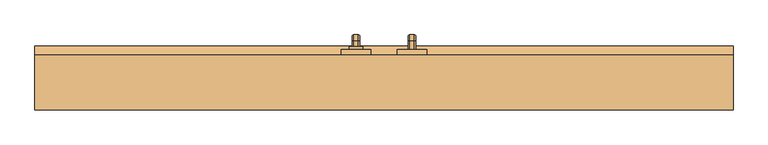
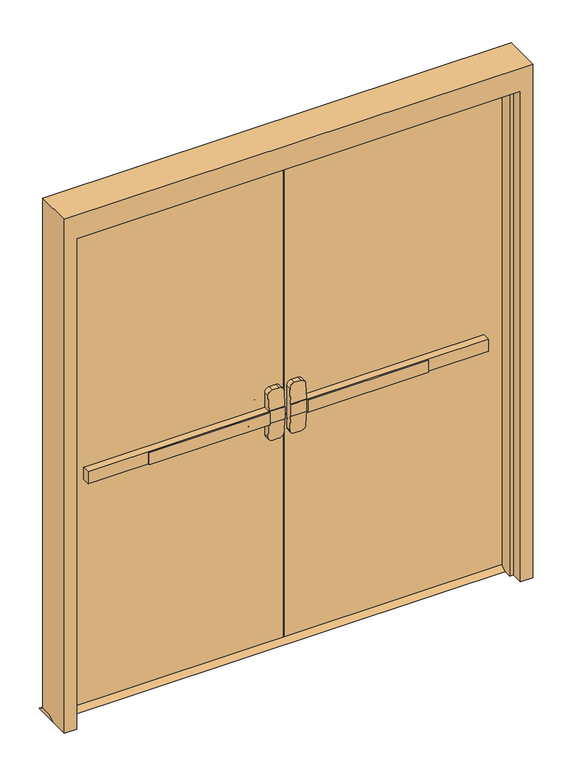
"""IFC4 building model written with IfcOpenShell, lengths in millimetres: door geometry, Дверь-Наружная-Двойная : Дверь-Наружная-Двойная."""

from ifc_helpers import new_model, si_unit, point, frame, frame_2d, origin, place, context, project, spatial, polyline, circle_curve, ellipse_curve, trimmed, segment, composite_curve, outline, extrude, faceted_brep, source, transform, mapped, element, save
from ifc_brep_helpers import plane_surface, cylinder_surface, revolved_surface, advanced_brep


def door_0e195155(model_context):
    return source(origin(), model_context, "Body", "SolidModel", [
        extrude(outline(polyline([(-566.1333333, -1.75), (-566.1333333, 4.6), (-76.2, 4.6), (-76.2, -1.75), (-566.1333333, -1.75)])), frame((0.0, 0.0, 974.6), z_axis=(0.0, 0.0, 1.0), x_axis=(1.0, 0.0, 0.0)), (0.0, 0.0, 1.0), 50.8),
        advanced_brep(
        [(-12.7, 4.6, 1025.4), (-76.2, 4.6, 1025.4), (-811.1, 4.6, 1025.4), (-811.1, 4.6, 974.6), (-76.2, 4.6, 974.6), (-12.7, 4.6, 974.6), (-811.1, 36.35, 1025.4), (-76.2, 36.35, 1025.4), (-76.2, 36.35, 1088.9), (-57.15, 36.35, 1107.95), (-31.75, 36.35, 1107.95), (-12.7, 36.35, 1088.9), (-12.7, 36.35, 911.1), (-31.75, 36.35, 892.05), (-57.15, 36.35, 892.05), (-76.2, 36.35, 911.1), (-76.2, 36.35, 974.6), (-811.1, 36.35, 974.6), (-12.7, 7.7752467, 1025.4), (-76.2, 7.7752467, 1025.4), (-12.7, 7.7752467, 974.6), (-12.7, 12.7854269, 911.1), (-12.7, 12.7854269, 1088.9), (-76.2, 7.7752467, 974.6), (-76.2, 12.7854269, 1088.9), (-76.2, 12.7854269, 911.1), (-57.15, 14.288481, 1107.95), (-31.75, 14.288481, 1107.95), (-31.75, 14.288481, 892.05), (-57.15, 14.288481, 892.05)],
        [
            (0, 1),
            (1, 2),
            (2, 3),
            (3, 4),
            (4, 5),
            (5, 0),
            (6, 7),
            (7, 8),
            (8, 9, circle_curve(frame((-57.15, 36.35, 1088.9), z_axis=(0.0, 1.0, 0.0), x_axis=(-1.0, 0.0, 0.0)), 19.05)),
            (9, 10),
            (10, 11, circle_curve(frame((-31.75, 36.35, 1088.9), z_axis=(0.0, 1.0, 0.0), x_axis=(-1.0, 0.0, 0.0)), 19.05)),
            (11, 12),
            (12, 13, circle_curve(frame((-31.75, 36.35, 911.1), z_axis=(0.0, 1.0, 0.0), x_axis=(-1.0, 0.0, 0.0)), 19.05)),
            (13, 14),
            (14, 15, circle_curve(frame((-57.15, 36.35, 911.1), z_axis=(0.0, 1.0, 0.0), x_axis=(-1.0, 0.0, 0.0)), 19.05)),
            (15, 16),
            (16, 17),
            (17, 6),
            (0, 18),
            (18, 19),
            (19, 7),
            (6, 2),
            (5, 20),
            (20, 21),
            (21, 12),
            (11, 22),
            (22, 18),
            (16, 23),
            (23, 20),
            (3, 17),
            (19, 24),
            (24, 8),
            (15, 25),
            (25, 23),
            (9, 26),
            (26, 27),
            (27, 10),
            (13, 28),
            (28, 29),
            (29, 14),
            (29, 25, ellipse_curve(frame((-57.15, 12.7854269, 911.1), z_axis=(0.0, 0.9969018152893365, 0.07865602756830282), x_axis=(0.0, -0.07865602756830208, 0.9969018152893365)), 19.1092038, 19.05)),
            (24, 26, ellipse_curve(frame((-57.15, 12.7854269, 1088.9), z_axis=(0.0, 0.9969018152893376, -0.07865602756828934), x_axis=(0.0, -0.078656027568288, -0.9969018152893377)), 19.1092038, 19.05)),
            (27, 22, ellipse_curve(frame((-31.75, 12.7854269, 1088.9), z_axis=(0.0, 0.9969018152893376, -0.07865602756828934), x_axis=(0.0, -0.078656027568288, -0.9969018152893377)), 19.1092038, 19.05)),
            (21, 28, ellipse_curve(frame((-31.75, 12.7854269, 911.1), z_axis=(0.0, 0.9969018152893365, 0.07865602756830282), x_axis=(0.0, -0.07865602756830208, 0.9969018152893365)), 19.1092038, 19.05)),
        ],
        [
            plane_surface(frame((-12.7, 4.6, 1025.4), z_axis=(0.0, -1.0, 0.0), x_axis=(1.0, 0.0, 0.0))),
            plane_surface(frame((-12.7, 36.35, 1025.4), z_axis=(0.0, 1.0, 0.0), x_axis=(-1.0, 0.0, 0.0))),
            plane_surface(frame((-811.1, 4.6, 1025.4), z_axis=(0.0, 0.0, 1.0), x_axis=(0.0, 1.0, 0.0))),
            plane_surface(frame((-12.7, 4.6, 1025.4), z_axis=(1.0, 0.0, 0.0), x_axis=(0.0, 1.0, 0.0))),
            plane_surface(frame((-12.7, 4.6, 974.6), z_axis=(0.0, 0.0, -1.0), x_axis=(0.0, 1.0, 0.0))),
            plane_surface(frame((-811.1, 4.6, 974.6), z_axis=(-1.0, 0.0, 0.0), x_axis=(0.0, 1.0, 0.0))),
            plane_surface(frame((-76.2, 7.7752467, 911.1), z_axis=(-1.0, 0.0, 0.0), x_axis=(0.0, 1.0, 0.0))),
            plane_surface(frame((-57.15, 7.7752467, 1107.95), z_axis=(0.0, 0.0, 1.0), x_axis=(0.0, 1.0, 0.0))),
            plane_surface(frame((-31.75, 7.7752467, 892.05), z_axis=(0.0, 0.0, -1.0), x_axis=(0.0, 1.0, 0.0))),
            cylinder_surface(frame((-57.15, 36.35, 911.1), z_axis=(0.0, -1.0, 0.0), x_axis=(-1.0, 0.0, 0.0)), 19.05),
            cylinder_surface(frame((-57.15, 36.35, 1088.9), z_axis=(0.0, -1.0, 0.0), x_axis=(-1.0, 0.0, 0.0)), 19.05),
            cylinder_surface(frame((-31.75, 36.35, 1088.9), z_axis=(0.0, -1.0, 0.0), x_axis=(-1.0, 0.0, 0.0)), 19.05),
            cylinder_surface(frame((-31.75, 36.35, 911.1), z_axis=(0.0, -1.0, 0.0), x_axis=(-1.0, 0.0, 0.0)), 19.05),
            plane_surface(frame((-76.2, 7.7752467, 1025.4), z_axis=(0.0, -0.9969018152893376, 0.07865602756828934), x_axis=(1.0, 0.0, 0.0))),
            plane_surface(frame((-76.2, 14.288481, 892.05), z_axis=(0.0, -0.9969018152893365, -0.07865602756830282), x_axis=(1.0, 0.0, 0.0))),
        ],
        [
            (0, [[1, 2, 3, 4, 5, 6]]),
            (1, [[7, 8, 9, 10, 11, 12, 13, 14, 15, 16, 17, 18]]),
            (2, [[-2, -1, 19, 20, 21, -7, 22]]),
            (3, [[23, 24, 25, -12, 26, 27, -19, -6]]),
            (4, [[-17, 28, 29, -23, -5, -4, 30]]),
            (5, [[-22, -18, -30, -3]]),
            (6, [[-21, 31, 32, -8]]),
            (6, [[33, 34, -28, -16]]),
            (7, [[35, 36, 37, -10]]),
            (8, [[38, 39, 40, -14]]),
            (9, [[-40, 41, -33, -15]]),
            (10, [[-32, 42, -35, -9]]),
            (11, [[-37, 43, -26, -11]]),
            (12, [[-25, 44, -38, -13]]),
            (13, [[-27, -43, -36, -42, -31, -20]]),
            (14, [[-29, -34, -41, -39, -44, -24]]),
        ],
    ),
        extrude(outline(polyline([(81.35, 15.0), (106.75, 0.0), (10.95, 0.0), (36.35, 15.0), (81.35, 15.0)])), frame((-950.0, 0.0, 0.0), z_axis=(1.0, 0.0, 0.0), x_axis=(0.0, 1.0, 0.0)), (0.0, 0.0, 1.0), 1900.0),
        extrude(outline(polyline([(566.1333333, -1.75), (76.2, -1.75), (76.2, 4.6), (566.1333333, 4.6), (566.1333333, -1.75)])), frame((0.0, 0.0, 974.6), z_axis=(0.0, 0.0, 1.0), x_axis=(1.0, 0.0, 0.0)), (0.0, 0.0, 1.0), 50.8),
        advanced_brep(
        [(12.7, 4.6, 1025.4), (12.7, 4.6, 974.6), (76.2, 4.6, 974.6), (811.1, 4.6, 974.6), (811.1, 4.6, 1025.4), (76.2, 4.6, 1025.4), (811.1, 36.35, 1025.4), (811.1, 36.35, 974.6), (76.2, 36.35, 974.6), (76.2, 36.35, 911.1), (57.15, 36.35, 892.05), (31.75, 36.35, 892.05), (12.7, 36.35, 911.1), (12.7, 36.35, 1088.9), (31.75, 36.35, 1107.95), (57.15, 36.35, 1107.95), (76.2, 36.35, 1088.9), (76.2, 36.35, 1025.4), (76.2, 7.7752467, 1025.4), (12.7, 7.7752467, 1025.4), (12.7, 12.7854269, 1088.9), (12.7, 12.7854269, 911.1), (12.7, 7.7752467, 974.6), (76.2, 7.7752467, 974.6), (76.2, 12.7854269, 911.1), (76.2, 12.7854269, 1088.9), (31.75, 14.288481, 1107.95), (57.15, 14.288481, 1107.95), (57.15, 14.288481, 892.05), (31.75, 14.288481, 892.05)],
        [
            (0, 1),
            (1, 2),
            (2, 3),
            (3, 4),
            (4, 5),
            (5, 0),
            (6, 7),
            (7, 8),
            (8, 9),
            (9, 10, circle_curve(frame((57.15, 36.35, 911.1), z_axis=(0.0, 1.0, 0.0), x_axis=(1.0, 0.0, 0.0)), 19.05)),
            (10, 11),
            (11, 12, circle_curve(frame((31.75, 36.35, 911.1), z_axis=(0.0, 1.0, 0.0), x_axis=(1.0, 0.0, 0.0)), 19.05)),
            (12, 13),
            (13, 14, circle_curve(frame((31.75, 36.35, 1088.9), z_axis=(0.0, 1.0, 0.0), x_axis=(1.0, 0.0, 0.0)), 19.05)),
            (14, 15),
            (15, 16, circle_curve(frame((57.15, 36.35, 1088.9), z_axis=(0.0, 1.0, 0.0), x_axis=(1.0, 0.0, 0.0)), 19.05)),
            (16, 17),
            (17, 6),
            (4, 6),
            (17, 18),
            (18, 19),
            (19, 0),
            (19, 20),
            (20, 13),
            (12, 21),
            (21, 22),
            (22, 1),
            (7, 3),
            (22, 23),
            (23, 8),
            (23, 24),
            (24, 9),
            (16, 25),
            (25, 18),
            (14, 26),
            (26, 27),
            (27, 15),
            (10, 28),
            (28, 29),
            (29, 11),
            (24, 28, ellipse_curve(frame((57.15, 12.7854269, 911.1), z_axis=(0.0, 0.9969018152893365, 0.07865602756830282), x_axis=(0.0, -0.07865602756830208, 0.9969018152893365)), 19.1092038, 19.05)),
            (27, 25, ellipse_curve(frame((57.15, 12.7854269, 1088.9), z_axis=(0.0, 0.9969018152893376, -0.07865602756828934), x_axis=(0.0, -0.078656027568288, -0.9969018152893377)), 19.1092038, 19.05)),
            (20, 26, ellipse_curve(frame((31.75, 12.7854269, 1088.9), z_axis=(0.0, 0.9969018152893376, -0.07865602756828934), x_axis=(0.0, -0.078656027568288, -0.9969018152893377)), 19.1092038, 19.05)),
            (29, 21, ellipse_curve(frame((31.75, 12.7854269, 911.1), z_axis=(0.0, 0.9969018152893365, 0.07865602756830282), x_axis=(0.0, -0.07865602756830208, 0.9969018152893365)), 19.1092038, 19.05)),
        ],
        [
            plane_surface(frame((12.7, 4.6, 1025.4), z_axis=(0.0, -1.0, 0.0), x_axis=(-1.0, 0.0, 0.0))),
            plane_surface(frame((12.7, 36.35, 1025.4), z_axis=(0.0, 1.0, 0.0), x_axis=(1.0, 0.0, 0.0))),
            plane_surface(frame((811.1, 4.6, 1025.4), z_axis=(0.0, 0.0, 1.0), x_axis=(0.0, 1.0, 0.0))),
            plane_surface(frame((12.7, 4.6, 1025.4), z_axis=(-1.0, 0.0, 0.0), x_axis=(0.0, 1.0, 0.0))),
            plane_surface(frame((12.7, 4.6, 974.6), z_axis=(0.0, 0.0, -1.0), x_axis=(0.0, 1.0, 0.0))),
            plane_surface(frame((811.1, 4.6, 974.6), z_axis=(1.0, 0.0, 0.0), x_axis=(0.0, 1.0, 0.0))),
            plane_surface(frame((76.2, 7.7752467, 911.1), z_axis=(1.0, 0.0, 0.0), x_axis=(0.0, 1.0, 0.0))),
            plane_surface(frame((57.15, 7.7752467, 1107.95), z_axis=(0.0, 0.0, 1.0), x_axis=(0.0, 1.0, 0.0))),
            plane_surface(frame((31.75, 7.7752467, 892.05), z_axis=(0.0, 0.0, -1.0), x_axis=(0.0, 1.0, 0.0))),
            cylinder_surface(frame((57.15, 36.35, 911.1), z_axis=(0.0, -1.0, 0.0), x_axis=(1.0, 0.0, 0.0)), 19.05),
            cylinder_surface(frame((57.15, 36.35, 1088.9), z_axis=(0.0, -1.0, 0.0), x_axis=(1.0, 0.0, 0.0)), 19.05),
            cylinder_surface(frame((31.75, 36.35, 1088.9), z_axis=(0.0, -1.0, 0.0), x_axis=(1.0, 0.0, 0.0)), 19.05),
            cylinder_surface(frame((31.75, 36.35, 911.1), z_axis=(0.0, -1.0, 0.0), x_axis=(1.0, 0.0, 0.0)), 19.05),
            plane_surface(frame((76.2, 7.7752467, 1025.4), z_axis=(0.0, -0.9969018152893376, 0.07865602756828934), x_axis=(-1.0, 0.0, 0.0))),
            plane_surface(frame((76.2, 14.288481, 892.05), z_axis=(0.0, -0.9969018152893365, -0.07865602756830282), x_axis=(-1.0, 0.0, 0.0))),
        ],
        [
            (0, [[1, 2, 3, 4, 5, 6]]),
            (1, [[7, 8, 9, 10, 11, 12, 13, 14, 15, 16, 17, 18]]),
            (2, [[19, -18, 20, 21, 22, -6, -5]]),
            (3, [[-1, -22, 23, 24, -13, 25, 26, 27]]),
            (4, [[28, -3, -2, -27, 29, 30, -8]]),
            (5, [[-4, -28, -7, -19]]),
            (6, [[-9, -30, 31, 32]]),
            (6, [[-17, 33, 34, -20]]),
            (7, [[-15, 35, 36, 37]]),
            (8, [[-11, 38, 39, 40]]),
            (9, [[-10, -32, 41, -38]]),
            (10, [[-16, -37, 42, -33]]),
            (11, [[-14, -24, 43, -35]]),
            (12, [[-12, -40, 44, -25]]),
            (13, [[-21, -34, -42, -36, -43, -23]]),
            (14, [[-26, -44, -39, -41, -31, -29]]),
        ],
    ),
        advanced_brep(
        [(66.2, 94.05, 1001.190625), (66.2, 94.05, 998.809375), (69.771875, 94.05, 995.2375), (82.6284594, 94.05, 995.2375), (86.2, 94.05, 998.8090406), (86.2, 94.05, 1001.190625), (82.628125, 94.05, 1004.7625), (69.771875, 94.05, 1004.7625), (66.2, 94.05, 874.609375), (69.771875, 94.05, 871.0375), (82.628125, 94.05, 871.0375), (86.2, 94.05, 874.609375), (86.2, 94.05, 876.9909594), (82.6284594, 94.05, 880.5625), (69.771875, 94.05, 880.5625), (66.2, 94.05, 876.990625), (66.2, 119.45, 1001.190625), (66.2, 133.340625, 987.3), (66.2, 133.340625, 888.5), (66.2, 119.45, 874.609375), (66.2, 119.45, 876.990625), (66.2, 130.959375, 888.5), (66.2, 130.959375, 987.3), (66.2, 119.45, 998.809375), (69.771875, 119.45, 995.2375), (82.6284594, 119.45, 995.2375), (86.2, 119.45, 998.8090406), (86.2, 130.9590406, 987.3), (86.2, 130.9590406, 888.5), (86.2, 119.45, 876.9909594), (86.2, 119.45, 874.609375), (86.2, 133.340625, 888.5), (86.2, 133.340625, 987.3), (86.2, 119.45, 1001.190625), (82.628125, 119.45, 1004.7625), (69.771875, 119.45, 1004.7625), (69.771875, 127.3875, 987.3), (82.6284594, 127.3875, 987.3), (82.628125, 136.9125, 987.3), (69.771875, 136.9125, 987.3), (69.771875, 127.3875, 888.5), (82.6284594, 127.3875, 888.5), (82.628125, 136.9125, 888.5), (69.771875, 136.9125, 888.5), (69.771875, 119.45, 880.5625), (82.6284594, 119.45, 880.5625), (82.628125, 119.45, 871.0375), (69.771875, 119.45, 871.0375)],
        [
            (0, 1),
            (1, 2, circle_curve(frame((69.771875, 94.05, 998.809375), z_axis=(0.0, -1.0, 0.0), x_axis=(0.0, 0.0, 1.0)), 3.571875)),
            (2, 3),
            (3, 4, circle_curve(frame((82.6284594, 94.05, 998.8090406), z_axis=(0.0, -1.0, 0.0), x_axis=(0.0, 0.0, 1.0)), 3.5715406)),
            (4, 5),
            (5, 6, circle_curve(frame((82.628125, 94.05, 1001.190625), z_axis=(0.0, -1.0, 0.0), x_axis=(0.0, 0.0, 1.0)), 3.571875)),
            (6, 7),
            (7, 0, circle_curve(frame((69.771875, 94.05, 1001.190625), z_axis=(0.0, -1.0, 0.0), x_axis=(0.0, 0.0, 1.0)), 3.571875)),
            (8, 9, circle_curve(frame((69.771875, 94.05, 874.609375), z_axis=(0.0, -1.0, 0.0), x_axis=(0.0, 0.0, -1.0)), 3.571875)),
            (9, 10),
            (10, 11, circle_curve(frame((82.628125, 94.05, 874.609375), z_axis=(0.0, -1.0, 0.0), x_axis=(0.0, 0.0, -1.0)), 3.571875)),
            (11, 12),
            (12, 13, circle_curve(frame((82.6284594, 94.05, 876.9909594), z_axis=(0.0, -1.0, 0.0), x_axis=(0.0, 0.0, -1.0)), 3.5715406)),
            (13, 14),
            (14, 15, circle_curve(frame((69.771875, 94.05, 876.990625), z_axis=(0.0, -1.0, 0.0), x_axis=(0.0, 0.0, -1.0)), 3.571875)),
            (15, 8),
            (0, 16),
            (16, 17, circle_curve(frame((66.2, 119.45, 987.3), z_axis=(-1.0, 0.0, 0.0), x_axis=(0.0, 0.0, 1.0)), 13.890625)),
            (17, 18),
            (18, 19, circle_curve(frame((66.2, 119.45, 888.5), z_axis=(-1.0, 0.0, 0.0), x_axis=(0.0, 1.0, 0.0)), 13.890625)),
            (19, 8),
            (15, 20),
            (20, 21, circle_curve(frame((66.2, 119.45, 888.5), z_axis=(1.0, 0.0, 0.0), x_axis=(0.0, 1.0, 0.0)), 11.509375)),
            (21, 22),
            (22, 23, circle_curve(frame((66.2, 119.45, 987.3), z_axis=(1.0, 0.0, 0.0), x_axis=(0.0, 0.0, 1.0)), 11.509375)),
            (23, 1),
            (23, 24, circle_curve(frame((69.771875, 119.45, 998.809375), z_axis=(0.0, -1.0, 0.0), x_axis=(0.0, 0.0, 1.0)), 3.571875)),
            (24, 2),
            (24, 25),
            (25, 3),
            (25, 26, circle_curve(frame((82.6284594, 119.45, 998.8090406), z_axis=(0.0, -1.0, 0.0), x_axis=(0.0, 0.0, 1.0)), 3.5715406)),
            (26, 4),
            (26, 27, circle_curve(frame((86.2, 119.45, 987.3), z_axis=(-1.0, 0.0, 0.0), x_axis=(0.0, 0.0, 1.0)), 11.5090406)),
            (27, 28),
            (28, 29, circle_curve(frame((86.2, 119.45, 888.5), z_axis=(-1.0, 0.0, 0.0), x_axis=(0.0, 1.0, 0.0)), 11.5090406)),
            (29, 12),
            (11, 30),
            (30, 31, circle_curve(frame((86.2, 119.45, 888.5), z_axis=(1.0, 0.0, 0.0), x_axis=(0.0, 1.0, 0.0)), 13.890625)),
            (31, 32),
            (32, 33, circle_curve(frame((86.2, 119.45, 987.3), z_axis=(1.0, 0.0, 0.0), x_axis=(0.0, 0.0, 1.0)), 13.890625)),
            (33, 5),
            (33, 34, circle_curve(frame((82.628125, 119.45, 1001.190625), z_axis=(0.0, -1.0, 0.0), x_axis=(0.0, 0.0, 1.0)), 3.571875)),
            (34, 6),
            (34, 35),
            (35, 7),
            (35, 16, circle_curve(frame((69.771875, 119.45, 1001.190625), z_axis=(0.0, -1.0, 0.0), x_axis=(0.0, 0.0, 1.0)), 3.571875)),
            (36, 24, circle_curve(frame((69.771875, 119.45, 987.3), z_axis=(1.0, 0.0, 0.0), x_axis=(0.0, 0.0, 1.0)), 7.9375)),
            (22, 36, circle_curve(frame((69.771875, 130.959375, 987.3), z_axis=(0.0, 0.0, 1.0), x_axis=(0.0, 1.0, 0.0)), 3.571875)),
            (37, 25, circle_curve(frame((82.6284594, 119.45, 987.3), z_axis=(1.0, 0.0, 0.0), x_axis=(0.0, 0.0, 1.0)), 7.9375)),
            (36, 37),
            (37, 27, circle_curve(frame((82.6284594, 130.9590406, 987.3), z_axis=(0.0, 0.0, 1.0), x_axis=(0.0, 1.0, 0.0)), 3.5715406)),
            (38, 34, circle_curve(frame((82.628125, 119.45, 987.3), z_axis=(1.0, 0.0, 0.0), x_axis=(0.0, 0.0, 1.0)), 17.4625)),
            (32, 38, circle_curve(frame((82.628125, 133.340625, 987.3), z_axis=(0.0, 0.0, 1.0), x_axis=(0.0, 1.0, 0.0)), 3.571875)),
            (39, 35, circle_curve(frame((69.771875, 119.45, 987.3), z_axis=(1.0, 0.0, 0.0), x_axis=(0.0, 0.0, 1.0)), 17.4625)),
            (38, 39),
            (39, 17, circle_curve(frame((69.771875, 133.340625, 987.3), z_axis=(0.0, 0.0, 1.0), x_axis=(0.0, 1.0, 0.0)), 3.571875)),
            (21, 40, circle_curve(frame((69.771875, 130.959375, 888.5), z_axis=(0.0, 0.0, 1.0), x_axis=(0.0, 1.0, 0.0)), 3.571875)),
            (40, 36),
            (40, 41),
            (41, 37),
            (41, 28, circle_curve(frame((82.6284594, 130.9590406, 888.5), z_axis=(0.0, 0.0, 1.0), x_axis=(0.0, 1.0, 0.0)), 3.5715406)),
            (31, 42, circle_curve(frame((82.628125, 133.340625, 888.5), z_axis=(0.0, 0.0, 1.0), x_axis=(0.0, 1.0, 0.0)), 3.571875)),
            (42, 38),
            (42, 43),
            (43, 39),
            (43, 18, circle_curve(frame((69.771875, 133.340625, 888.5), z_axis=(0.0, 0.0, 1.0), x_axis=(0.0, 1.0, 0.0)), 3.571875)),
            (44, 40, circle_curve(frame((69.771875, 119.45, 888.5), z_axis=(1.0, 0.0, 0.0), x_axis=(0.0, 1.0, 0.0)), 7.9375)),
            (20, 44, circle_curve(frame((69.771875, 119.45, 876.990625), z_axis=(0.0, 1.0, 0.0), x_axis=(0.0, 0.0, -1.0)), 3.571875)),
            (45, 41, circle_curve(frame((82.6284594, 119.45, 888.5), z_axis=(1.0, 0.0, 0.0), x_axis=(0.0, 1.0, 0.0)), 7.9375)),
            (44, 45),
            (45, 29, circle_curve(frame((82.6284594, 119.45, 876.9909594), z_axis=(0.0, 1.0, 0.0), x_axis=(0.0, 0.0, -1.0)), 3.5715406)),
            (46, 42, circle_curve(frame((82.628125, 119.45, 888.5), z_axis=(1.0, 0.0, 0.0), x_axis=(0.0, 1.0, 0.0)), 17.4625)),
            (30, 46, circle_curve(frame((82.628125, 119.45, 874.609375), z_axis=(0.0, 1.0, 0.0), x_axis=(0.0, 0.0, -1.0)), 3.571875)),
            (47, 43, circle_curve(frame((69.771875, 119.45, 888.5), z_axis=(1.0, 0.0, 0.0), x_axis=(0.0, 1.0, 0.0)), 17.4625)),
            (46, 47),
            (47, 19, circle_curve(frame((69.771875, 119.45, 874.609375), z_axis=(0.0, 1.0, 0.0), x_axis=(0.0, 0.0, -1.0)), 3.571875)),
            (14, 44),
            (13, 45),
            (10, 46),
            (9, 47),
        ],
        [
            plane_surface(frame((76.2, 94.05, 1000.0), z_axis=(0.0, -1.0, 0.0), x_axis=(1.0, 0.0, 0.0))),
            plane_surface(frame((76.2, 94.05, 875.8), z_axis=(0.0, -1.0, 0.0), x_axis=(1.0, 0.0, 0.0))),
            plane_surface(frame((66.2, 94.05, 1001.190625), z_axis=(-1.0, 0.0, 0.0), x_axis=(0.0, 1.0, 0.0))),
            cylinder_surface(frame((69.771875, 94.05, 998.809375), z_axis=(0.0, -1.0, 0.0), x_axis=(0.0, 0.0, 1.0)), 3.571875),
            plane_surface(frame((69.771875, 94.05, 995.2375), z_axis=(0.0, 0.0, -1.0), x_axis=(0.0, 1.0, 0.0))),
            cylinder_surface(frame((82.6284594, 94.05, 998.8090406), z_axis=(0.0, -1.0, 0.0), x_axis=(0.0, 0.0, 1.0)), 3.5715406),
            plane_surface(frame((86.2, 94.05, 998.8090406), z_axis=(1.0, 0.0, 0.0), x_axis=(0.0, 1.0, 0.0))),
            cylinder_surface(frame((82.628125, 94.05, 1001.190625), z_axis=(0.0, -1.0, 0.0), x_axis=(0.0, 0.0, 1.0)), 3.571875),
            plane_surface(frame((82.628125, 94.05, 1004.7625), z_axis=(0.0, 0.0, 1.0), x_axis=(0.0, 1.0, 0.0))),
            cylinder_surface(frame((69.771875, 94.05, 1001.190625), z_axis=(0.0, -1.0, 0.0), x_axis=(0.0, 0.0, 1.0)), 3.571875),
            revolved_surface(trimmed(ellipse_curve(frame((69.771875, 119.45, 998.809375), z_axis=(0.0, -1.0, 0.0), x_axis=(0.0, 0.0, 1.0)), 3.571875, 3.571875), [point((66.2, 119.45, 998.809375))], [point((69.771875, 119.45, 995.2375))], True, "CARTESIAN"), (76.2, 119.45, 987.3), (-1.0, 0.0, 0.0)),
            revolved_surface(polyline([(69.771875, 119.45, 995.2375), (82.6284594, 119.45, 995.2375)]), (76.2, 119.45, 987.3), (-1.0, 0.0, 0.0)),
            revolved_surface(trimmed(ellipse_curve(frame((82.6284594, 119.45, 998.8090406), z_axis=(0.0, -1.0, 0.0), x_axis=(0.0, 0.0, 1.0)), 3.5715406, 3.5715406), [point((82.6284594, 119.45, 995.2375))], [point((86.2, 119.45, 998.8090406))], True, "CARTESIAN"), (76.2, 119.45, 987.3), (-1.0, 0.0, 0.0)),
            revolved_surface(trimmed(ellipse_curve(frame((82.628125, 119.45, 1001.190625), z_axis=(0.0, -1.0, 0.0), x_axis=(0.0, 0.0, 1.0)), 3.571875, 3.571875), [point((86.2, 119.45, 1001.190625))], [point((82.628125, 119.45, 1004.7625))], True, "CARTESIAN"), (76.2, 119.45, 987.3), (-1.0, 0.0, 0.0)),
            cylinder_surface(frame((76.2, 119.45, 987.3), z_axis=(-1.0, 0.0, 0.0), x_axis=(0.0, 0.0, 1.0)), 17.4625),
            revolved_surface(trimmed(ellipse_curve(frame((69.771875, 119.45, 1001.190625), z_axis=(0.0, -1.0, 0.0), x_axis=(0.0, 0.0, 1.0)), 3.571875, 3.571875), [point((69.771875, 119.45, 1004.7625))], [point((66.2, 119.45, 1001.190625))], True, "CARTESIAN"), (76.2, 119.45, 987.3), (-1.0, 0.0, 0.0)),
            cylinder_surface(frame((69.771875, 130.959375, 987.3), z_axis=(0.0, 0.0, 1.0), x_axis=(0.0, 1.0, 0.0)), 3.571875),
            plane_surface(frame((69.771875, 127.3875, 987.3), z_axis=(0.0, -1.0, 0.0), x_axis=(0.0, 0.0, -1.0))),
            cylinder_surface(frame((82.6284594, 130.9590406, 987.3), z_axis=(0.0, 0.0, 1.0), x_axis=(0.0, 1.0, 0.0)), 3.5715406),
            cylinder_surface(frame((82.628125, 133.340625, 987.3), z_axis=(0.0, 0.0, 1.0), x_axis=(0.0, 1.0, 0.0)), 3.571875),
            plane_surface(frame((82.628125, 136.9125, 987.3), z_axis=(0.0, 1.0, 0.0), x_axis=(0.0, 0.0, -1.0))),
            cylinder_surface(frame((69.771875, 133.340625, 987.3), z_axis=(0.0, 0.0, 1.0), x_axis=(0.0, 1.0, 0.0)), 3.571875),
            revolved_surface(trimmed(ellipse_curve(frame((69.771875, 130.959375, 888.5), z_axis=(0.0, 0.0, 1.0), x_axis=(0.0, 1.0, 0.0)), 3.571875, 3.571875), [point((66.2, 130.959375, 888.5))], [point((69.771875, 127.3875, 888.5))], True, "CARTESIAN"), (76.2, 119.45, 888.5), (-1.0, 0.0, 0.0)),
            revolved_surface(polyline([(69.771875, 127.3875, 888.5), (82.6284594, 127.3875, 888.5)]), (76.2, 119.45, 888.5), (-1.0, 0.0, 0.0)),
            revolved_surface(trimmed(ellipse_curve(frame((82.6284594, 130.9590406, 888.5), z_axis=(0.0, 0.0, 1.0), x_axis=(0.0, 1.0, 0.0)), 3.5715406, 3.5715406), [point((82.6284594, 127.3875, 888.5))], [point((86.2, 130.9590406, 888.5))], True, "CARTESIAN"), (76.2, 119.45, 888.5), (-1.0, 0.0, 0.0)),
            revolved_surface(trimmed(ellipse_curve(frame((82.628125, 133.340625, 888.5), z_axis=(0.0, 0.0, 1.0), x_axis=(0.0, 1.0, 0.0)), 3.571875, 3.571875), [point((86.2, 133.340625, 888.5))], [point((82.628125, 136.9125, 888.5))], True, "CARTESIAN"), (76.2, 119.45, 888.5), (-1.0, 0.0, 0.0)),
            cylinder_surface(frame((76.2, 119.45, 888.5), z_axis=(-1.0, 0.0, 0.0), x_axis=(0.0, 1.0, 0.0)), 17.4625),
            revolved_surface(trimmed(ellipse_curve(frame((69.771875, 133.340625, 888.5), z_axis=(0.0, 0.0, 1.0), x_axis=(0.0, 1.0, 0.0)), 3.571875, 3.571875), [point((69.771875, 136.9125, 888.5))], [point((66.2, 133.340625, 888.5))], True, "CARTESIAN"), (76.2, 119.45, 888.5), (-1.0, 0.0, 0.0)),
            cylinder_surface(frame((69.771875, 119.45, 876.990625), z_axis=(0.0, 1.0, 0.0), x_axis=(0.0, 0.0, -1.0)), 3.571875),
            plane_surface(frame((69.771875, 119.45, 880.5625), z_axis=(0.0, 0.0, 1.0), x_axis=(0.0, -1.0, 0.0))),
            cylinder_surface(frame((82.6284594, 119.45, 876.9909594), z_axis=(0.0, 1.0, 0.0), x_axis=(0.0, 0.0, -1.0)), 3.5715406),
            cylinder_surface(frame((82.628125, 119.45, 874.609375), z_axis=(0.0, 1.0, 0.0), x_axis=(0.0, 0.0, -1.0)), 3.571875),
            plane_surface(frame((82.628125, 119.45, 871.0375), z_axis=(0.0, 0.0, -1.0), x_axis=(0.0, -1.0, 0.0))),
            cylinder_surface(frame((69.771875, 119.45, 874.609375), z_axis=(0.0, 1.0, 0.0), x_axis=(0.0, 0.0, -1.0)), 3.571875),
        ],
        [
            (0, [[1, 2, 3, 4, 5, 6, 7, 8]]),
            (1, [[9, 10, 11, 12, 13, 14, 15, 16]]),
            (2, [[-1, 17, 18, 19, 20, 21, -16, 22, 23, 24, 25, 26]]),
            (3, [[-2, -26, 27, 28]]),
            (4, [[-3, -28, 29, 30]]),
            (5, [[-4, -30, 31, 32]]),
            (6, [[-5, -32, 33, 34, 35, 36, -12, 37, 38, 39, 40, 41]]),
            (7, [[-6, -41, 42, 43]]),
            (8, [[-7, -43, 44, 45]]),
            (9, [[-8, -45, 46, -17]]),
            (10, [[47, -27, -25, 48]]),
            (11, [[49, -29, -47, 50]]),
            (12, [[-33, -31, -49, 51]]),
            (13, [[52, -42, -40, 53]]),
            (14, [[54, -44, -52, 55]]),
            (15, [[-18, -46, -54, 56]]),
            (16, [[-48, -24, 57, 58]]),
            (17, [[-50, -58, 59, 60]]),
            (18, [[-51, -60, 61, -34]]),
            (19, [[-53, -39, 62, 63]]),
            (20, [[-55, -63, 64, 65]]),
            (21, [[-56, -65, 66, -19]]),
            (22, [[67, -57, -23, 68]]),
            (23, [[69, -59, -67, 70]]),
            (24, [[-35, -61, -69, 71]]),
            (25, [[72, -62, -38, 73]]),
            (26, [[74, -64, -72, 75]]),
            (27, [[-20, -66, -74, 76]]),
            (28, [[-68, -22, -15, 77]]),
            (29, [[-70, -77, -14, 78]]),
            (30, [[-71, -78, -13, -36]]),
            (31, [[-73, -37, -11, 79]]),
            (32, [[-75, -79, -10, 80]]),
            (33, [[-76, -80, -9, -21]]),
        ],
    ),
        extrude(outline(composite_curve([segment(trimmed(circle_curve(frame_2d((1094.2338574, 76.2)), 90.1286291), [point((1175.0, 116.2))], [point((1175.0, 36.2))], False, "CARTESIAN"), True, "CONTINUOUS"), segment(polyline([(1175.0, 36.2), (825.0, 36.2)]), True, "CONTINUOUS"), segment(trimmed(circle_curve(frame_2d((905.7661426, 76.2)), 90.1286291), [point((825.0, 36.2))], [point((825.0, 116.2))], False, "CARTESIAN"), True, "CONTINUOUS"), segment(polyline([(825.0, 116.2), (1175.0, 116.2)]), True, "CONTINUOUS")], self_intersect=False)), frame((0.0, 81.35, 0.0), z_axis=(0.0, 1.0, 0.0), x_axis=(0.0, 0.0, 1.0)), (0.0, 0.0, 1.0), 15.0),
        advanced_brep(
        [(-86.2, 94.05, 1001.190625), (-86.2, 94.05, 998.809375), (-82.628125, 94.05, 995.2375), (-69.7715406, 94.05, 995.2375), (-66.2, 94.05, 998.8090406), (-66.2, 94.05, 1001.190625), (-69.771875, 94.05, 1004.7625), (-82.628125, 94.05, 1004.7625), (-86.2, 94.05, 874.609375), (-82.628125, 94.05, 871.0375), (-69.771875, 94.05, 871.0375), (-66.2, 94.05, 874.609375), (-66.2, 94.05, 876.9909594), (-69.7715406, 94.05, 880.5625), (-82.628125, 94.05, 880.5625), (-86.2, 94.05, 876.990625), (-86.2, 119.45, 1001.190625), (-86.2, 133.340625, 987.3), (-86.2, 133.340625, 888.5), (-86.2, 119.45, 874.609375), (-86.2, 119.45, 876.990625), (-86.2, 130.959375, 888.5), (-86.2, 130.959375, 987.3), (-86.2, 119.45, 998.809375), (-82.628125, 119.45, 995.2375), (-69.7715406, 119.45, 995.2375), (-66.2, 119.45, 998.8090406), (-66.2, 130.9590406, 987.3), (-66.2, 130.9590406, 888.5), (-66.2, 119.45, 876.9909594), (-66.2, 119.45, 874.609375), (-66.2, 133.340625, 888.5), (-66.2, 133.340625, 987.3), (-66.2, 119.45, 1001.190625), (-69.771875, 119.45, 1004.7625), (-82.628125, 119.45, 1004.7625), (-82.628125, 127.3875, 987.3), (-69.7715406, 127.3875, 987.3), (-69.771875, 136.9125, 987.3), (-82.628125, 136.9125, 987.3), (-82.628125, 127.3875, 888.5), (-69.7715406, 127.3875, 888.5), (-69.771875, 136.9125, 888.5), (-82.628125, 136.9125, 888.5), (-82.628125, 119.45, 880.5625), (-69.7715406, 119.45, 880.5625), (-69.771875, 119.45, 871.0375), (-82.628125, 119.45, 871.0375)],
        [
            (0, 1),
            (1, 2, circle_curve(frame((-82.628125, 94.05, 998.809375), z_axis=(0.0, -1.0, 0.0), x_axis=(0.0, 0.0, 1.0)), 3.571875)),
            (2, 3),
            (3, 4, circle_curve(frame((-69.7715406, 94.05, 998.8090406), z_axis=(0.0, -1.0, 0.0), x_axis=(0.0, 0.0, 1.0)), 3.5715406)),
            (4, 5),
            (5, 6, circle_curve(frame((-69.771875, 94.05, 1001.190625), z_axis=(0.0, -1.0, 0.0), x_axis=(0.0, 0.0, 1.0)), 3.571875)),
            (6, 7),
            (7, 0, circle_curve(frame((-82.628125, 94.05, 1001.190625), z_axis=(0.0, -1.0, 0.0), x_axis=(0.0, 0.0, 1.0)), 3.571875)),
            (8, 9, circle_curve(frame((-82.628125, 94.05, 874.609375), z_axis=(0.0, -1.0, 0.0), x_axis=(0.0, 0.0, -1.0)), 3.571875)),
            (9, 10),
            (10, 11, circle_curve(frame((-69.771875, 94.05, 874.609375), z_axis=(0.0, -1.0, 0.0), x_axis=(0.0, 0.0, -1.0)), 3.571875)),
            (11, 12),
            (12, 13, circle_curve(frame((-69.7715406, 94.05, 876.9909594), z_axis=(0.0, -1.0, 0.0), x_axis=(0.0, 0.0, -1.0)), 3.5715406)),
            (13, 14),
            (14, 15, circle_curve(frame((-82.628125, 94.05, 876.990625), z_axis=(0.0, -1.0, 0.0), x_axis=(0.0, 0.0, -1.0)), 3.571875)),
            (15, 8),
            (0, 16),
            (16, 17, circle_curve(frame((-86.2, 119.45, 987.3), z_axis=(-1.0, 0.0, 0.0), x_axis=(0.0, 0.0, 1.0)), 13.890625)),
            (17, 18),
            (18, 19, circle_curve(frame((-86.2, 119.45, 888.5), z_axis=(-1.0, 0.0, 0.0), x_axis=(0.0, 1.0, 0.0)), 13.890625)),
            (19, 8),
            (15, 20),
            (20, 21, circle_curve(frame((-86.2, 119.45, 888.5), z_axis=(1.0, 0.0, 0.0), x_axis=(0.0, 1.0, 0.0)), 11.509375)),
            (21, 22),
            (22, 23, circle_curve(frame((-86.2, 119.45, 987.3), z_axis=(1.0, 0.0, 0.0), x_axis=(0.0, 0.0, 1.0)), 11.509375)),
            (23, 1),
            (23, 24, circle_curve(frame((-82.628125, 119.45, 998.809375), z_axis=(0.0, -1.0, 0.0), x_axis=(0.0, 0.0, 1.0)), 3.571875)),
            (24, 2),
            (24, 25),
            (25, 3),
            (25, 26, circle_curve(frame((-69.7715406, 119.45, 998.8090406), z_axis=(0.0, -1.0, 0.0), x_axis=(0.0, 0.0, 1.0)), 3.5715406)),
            (26, 4),
            (26, 27, circle_curve(frame((-66.2, 119.45, 987.3), z_axis=(-1.0, 0.0, 0.0), x_axis=(0.0, 0.0, 1.0)), 11.5090406)),
            (27, 28),
            (28, 29, circle_curve(frame((-66.2, 119.45, 888.5), z_axis=(-1.0, 0.0, 0.0), x_axis=(0.0, 1.0, 0.0)), 11.5090406)),
            (29, 12),
            (11, 30),
            (30, 31, circle_curve(frame((-66.2, 119.45, 888.5), z_axis=(1.0, 0.0, 0.0), x_axis=(0.0, 1.0, 0.0)), 13.890625)),
            (31, 32),
            (32, 33, circle_curve(frame((-66.2, 119.45, 987.3), z_axis=(1.0, 0.0, 0.0), x_axis=(0.0, 0.0, 1.0)), 13.890625)),
            (33, 5),
            (33, 34, circle_curve(frame((-69.771875, 119.45, 1001.190625), z_axis=(0.0, -1.0, 0.0), x_axis=(0.0, 0.0, 1.0)), 3.571875)),
            (34, 6),
            (34, 35),
            (35, 7),
            (35, 16, circle_curve(frame((-82.628125, 119.45, 1001.190625), z_axis=(0.0, -1.0, 0.0), x_axis=(0.0, 0.0, 1.0)), 3.571875)),
            (36, 24, circle_curve(frame((-82.628125, 119.45, 987.3), z_axis=(1.0, 0.0, 0.0), x_axis=(0.0, 0.0, 1.0)), 7.9375)),
            (22, 36, circle_curve(frame((-82.628125, 130.959375, 987.3), z_axis=(0.0, 0.0, 1.0), x_axis=(0.0, 1.0, 0.0)), 3.571875)),
            (37, 25, circle_curve(frame((-69.7715406, 119.45, 987.3), z_axis=(1.0, 0.0, 0.0), x_axis=(0.0, 0.0, 1.0)), 7.9375)),
            (36, 37),
            (37, 27, circle_curve(frame((-69.7715406, 130.9590406, 987.3), z_axis=(0.0, 0.0, 1.0), x_axis=(0.0, 1.0, 0.0)), 3.5715406)),
            (38, 34, circle_curve(frame((-69.771875, 119.45, 987.3), z_axis=(1.0, 0.0, 0.0), x_axis=(0.0, 0.0, 1.0)), 17.4625)),
            (32, 38, circle_curve(frame((-69.771875, 133.340625, 987.3), z_axis=(0.0, 0.0, 1.0), x_axis=(0.0, 1.0, 0.0)), 3.571875)),
            (39, 35, circle_curve(frame((-82.628125, 119.45, 987.3), z_axis=(1.0, 0.0, 0.0), x_axis=(0.0, 0.0, 1.0)), 17.4625)),
            (38, 39),
            (39, 17, circle_curve(frame((-82.628125, 133.340625, 987.3), z_axis=(0.0, 0.0, 1.0), x_axis=(0.0, 1.0, 0.0)), 3.571875)),
            (21, 40, circle_curve(frame((-82.628125, 130.959375, 888.5), z_axis=(0.0, 0.0, 1.0), x_axis=(0.0, 1.0, 0.0)), 3.571875)),
            (40, 36),
            (40, 41),
            (41, 37),
            (41, 28, circle_curve(frame((-69.7715406, 130.9590406, 888.5), z_axis=(0.0, 0.0, 1.0), x_axis=(0.0, 1.0, 0.0)), 3.5715406)),
            (31, 42, circle_curve(frame((-69.771875, 133.340625, 888.5), z_axis=(0.0, 0.0, 1.0), x_axis=(0.0, 1.0, 0.0)), 3.571875)),
            (42, 38),
            (42, 43),
            (43, 39),
            (43, 18, circle_curve(frame((-82.628125, 133.340625, 888.5), z_axis=(0.0, 0.0, 1.0), x_axis=(0.0, 1.0, 0.0)), 3.571875)),
            (44, 40, circle_curve(frame((-82.628125, 119.45, 888.5), z_axis=(1.0, 0.0, 0.0), x_axis=(0.0, 1.0, 0.0)), 7.9375)),
            (20, 44, circle_curve(frame((-82.628125, 119.45, 876.990625), z_axis=(0.0, 1.0, 0.0), x_axis=(0.0, 0.0, -1.0)), 3.571875)),
            (45, 41, circle_curve(frame((-69.7715406, 119.45, 888.5), z_axis=(1.0, 0.0, 0.0), x_axis=(0.0, 1.0, 0.0)), 7.9375)),
            (44, 45),
            (45, 29, circle_curve(frame((-69.7715406, 119.45, 876.9909594), z_axis=(0.0, 1.0, 0.0), x_axis=(0.0, 0.0, -1.0)), 3.5715406)),
            (46, 42, circle_curve(frame((-69.771875, 119.45, 888.5), z_axis=(1.0, 0.0, 0.0), x_axis=(0.0, 1.0, 0.0)), 17.4625)),
            (30, 46, circle_curve(frame((-69.771875, 119.45, 874.609375), z_axis=(0.0, 1.0, 0.0), x_axis=(0.0, 0.0, -1.0)), 3.571875)),
            (47, 43, circle_curve(frame((-82.628125, 119.45, 888.5), z_axis=(1.0, 0.0, 0.0), x_axis=(0.0, 1.0, 0.0)), 17.4625)),
            (46, 47),
            (47, 19, circle_curve(frame((-82.628125, 119.45, 874.609375), z_axis=(0.0, 1.0, 0.0), x_axis=(0.0, 0.0, -1.0)), 3.571875)),
            (14, 44),
            (13, 45),
            (10, 46),
            (9, 47),
        ],
        [
            plane_surface(frame((-76.2, 94.05, 1000.0), z_axis=(0.0, -1.0, 0.0), x_axis=(1.0, 0.0, 0.0))),
            plane_surface(frame((-76.2, 94.05, 875.8), z_axis=(0.0, -1.0, 0.0), x_axis=(1.0, 0.0, 0.0))),
            plane_surface(frame((-86.2, 94.05, 1001.190625), z_axis=(-1.0, 0.0, 0.0), x_axis=(0.0, 1.0, 0.0))),
            cylinder_surface(frame((-82.628125, 94.05, 998.809375), z_axis=(0.0, -1.0, 0.0), x_axis=(0.0, 0.0, 1.0)), 3.571875),
            plane_surface(frame((-82.628125, 94.05, 995.2375), z_axis=(0.0, 0.0, -1.0), x_axis=(0.0, 1.0, 0.0))),
            cylinder_surface(frame((-69.7715406, 94.05, 998.8090406), z_axis=(0.0, -1.0, 0.0), x_axis=(0.0, 0.0, 1.0)), 3.5715406),
            plane_surface(frame((-66.2, 94.05, 998.8090406), z_axis=(1.0, 0.0, 0.0), x_axis=(0.0, 1.0, 0.0))),
            cylinder_surface(frame((-69.771875, 94.05, 1001.190625), z_axis=(0.0, -1.0, 0.0), x_axis=(0.0, 0.0, 1.0)), 3.571875),
            plane_surface(frame((-69.771875, 94.05, 1004.7625), z_axis=(0.0, 0.0, 1.0), x_axis=(0.0, 1.0, 0.0))),
            cylinder_surface(frame((-82.628125, 94.05, 1001.190625), z_axis=(0.0, -1.0, 0.0), x_axis=(0.0, 0.0, 1.0)), 3.571875),
            revolved_surface(trimmed(ellipse_curve(frame((-82.628125, 119.45, 998.809375), z_axis=(0.0, -1.0, 0.0), x_axis=(0.0, 0.0, 1.0)), 3.571875, 3.571875), [point((-86.2, 119.45, 998.809375))], [point((-82.628125, 119.45, 995.2375))], True, "CARTESIAN"), (-76.2, 119.45, 987.3), (-1.0, 0.0, 0.0)),
            revolved_surface(polyline([(-82.628125, 119.45, 995.2375), (-69.7715406, 119.45, 995.2375)]), (-76.2, 119.45, 987.3), (-1.0, 0.0, 0.0)),
            revolved_surface(trimmed(ellipse_curve(frame((-69.7715406, 119.45, 998.8090406), z_axis=(0.0, -1.0, 0.0), x_axis=(0.0, 0.0, 1.0)), 3.5715406, 3.5715406), [point((-69.7715406, 119.45, 995.2375))], [point((-66.2, 119.45, 998.8090406))], True, "CARTESIAN"), (-76.2, 119.45, 987.3), (-1.0, 0.0, 0.0)),
            revolved_surface(trimmed(ellipse_curve(frame((-69.771875, 119.45, 1001.190625), z_axis=(0.0, -1.0, 0.0), x_axis=(0.0, 0.0, 1.0)), 3.571875, 3.571875), [point((-66.2, 119.45, 1001.190625))], [point((-69.771875, 119.45, 1004.7625))], True, "CARTESIAN"), (-76.2, 119.45, 987.3), (-1.0, 0.0, 0.0)),
            cylinder_surface(frame((-76.2, 119.45, 987.3), z_axis=(-1.0, 0.0, 0.0), x_axis=(0.0, 0.0, 1.0)), 17.4625),
            revolved_surface(trimmed(ellipse_curve(frame((-82.628125, 119.45, 1001.190625), z_axis=(0.0, -1.0, 0.0), x_axis=(0.0, 0.0, 1.0)), 3.571875, 3.571875), [point((-82.628125, 119.45, 1004.7625))], [point((-86.2, 119.45, 1001.190625))], True, "CARTESIAN"), (-76.2, 119.45, 987.3), (-1.0, 0.0, 0.0)),
            cylinder_surface(frame((-82.628125, 130.959375, 987.3), z_axis=(0.0, 0.0, 1.0), x_axis=(0.0, 1.0, 0.0)), 3.571875),
            plane_surface(frame((-82.628125, 127.3875, 987.3), z_axis=(0.0, -1.0, 0.0), x_axis=(0.0, 0.0, -1.0))),
            cylinder_surface(frame((-69.7715406, 130.9590406, 987.3), z_axis=(0.0, 0.0, 1.0), x_axis=(0.0, 1.0, 0.0)), 3.5715406),
            cylinder_surface(frame((-69.771875, 133.340625, 987.3), z_axis=(0.0, 0.0, 1.0), x_axis=(0.0, 1.0, 0.0)), 3.571875),
            plane_surface(frame((-69.771875, 136.9125, 987.3), z_axis=(0.0, 1.0, 0.0), x_axis=(0.0, 0.0, -1.0))),
            cylinder_surface(frame((-82.628125, 133.340625, 987.3), z_axis=(0.0, 0.0, 1.0), x_axis=(0.0, 1.0, 0.0)), 3.571875),
            revolved_surface(trimmed(ellipse_curve(frame((-82.628125, 130.959375, 888.5), z_axis=(0.0, 0.0, 1.0), x_axis=(0.0, 1.0, 0.0)), 3.571875, 3.571875), [point((-86.2, 130.959375, 888.5))], [point((-82.628125, 127.3875, 888.5))], True, "CARTESIAN"), (-76.2, 119.45, 888.5), (-1.0, 0.0, 0.0)),
            revolved_surface(polyline([(-82.628125, 127.3875, 888.5), (-69.7715406, 127.3875, 888.5)]), (-76.2, 119.45, 888.5), (-1.0, 0.0, 0.0)),
            revolved_surface(trimmed(ellipse_curve(frame((-69.7715406, 130.9590406, 888.5), z_axis=(0.0, 0.0, 1.0), x_axis=(0.0, 1.0, 0.0)), 3.5715406, 3.5715406), [point((-69.7715406, 127.3875, 888.5))], [point((-66.2, 130.9590406, 888.5))], True, "CARTESIAN"), (-76.2, 119.45, 888.5), (-1.0, 0.0, 0.0)),
            revolved_surface(trimmed(ellipse_curve(frame((-69.771875, 133.340625, 888.5), z_axis=(0.0, 0.0, 1.0), x_axis=(0.0, 1.0, 0.0)), 3.571875, 3.571875), [point((-66.2, 133.340625, 888.5))], [point((-69.771875, 136.9125, 888.5))], True, "CARTESIAN"), (-76.2, 119.45, 888.5), (-1.0, 0.0, 0.0)),
            cylinder_surface(frame((-76.2, 119.45, 888.5), z_axis=(-1.0, 0.0, 0.0), x_axis=(0.0, 1.0, 0.0)), 17.4625),
            revolved_surface(trimmed(ellipse_curve(frame((-82.628125, 133.340625, 888.5), z_axis=(0.0, 0.0, 1.0), x_axis=(0.0, 1.0, 0.0)), 3.571875, 3.571875), [point((-82.628125, 136.9125, 888.5))], [point((-86.2, 133.340625, 888.5))], True, "CARTESIAN"), (-76.2, 119.45, 888.5), (-1.0, 0.0, 0.0)),
            cylinder_surface(frame((-82.628125, 119.45, 876.990625), z_axis=(0.0, 1.0, 0.0), x_axis=(0.0, 0.0, -1.0)), 3.571875),
            plane_surface(frame((-82.628125, 119.45, 880.5625), z_axis=(0.0, 0.0, 1.0), x_axis=(0.0, -1.0, 0.0))),
            cylinder_surface(frame((-69.7715406, 119.45, 876.9909594), z_axis=(0.0, 1.0, 0.0), x_axis=(0.0, 0.0, -1.0)), 3.5715406),
            cylinder_surface(frame((-69.771875, 119.45, 874.609375), z_axis=(0.0, 1.0, 0.0), x_axis=(0.0, 0.0, -1.0)), 3.571875),
            plane_surface(frame((-69.771875, 119.45, 871.0375), z_axis=(0.0, 0.0, -1.0), x_axis=(0.0, -1.0, 0.0))),
            cylinder_surface(frame((-82.628125, 119.45, 874.609375), z_axis=(0.0, 1.0, 0.0), x_axis=(0.0, 0.0, -1.0)), 3.571875),
        ],
        [
            (0, [[1, 2, 3, 4, 5, 6, 7, 8]]),
            (1, [[9, 10, 11, 12, 13, 14, 15, 16]]),
            (2, [[-1, 17, 18, 19, 20, 21, -16, 22, 23, 24, 25, 26]]),
            (3, [[-2, -26, 27, 28]]),
            (4, [[-3, -28, 29, 30]]),
            (5, [[-4, -30, 31, 32]]),
            (6, [[-5, -32, 33, 34, 35, 36, -12, 37, 38, 39, 40, 41]]),
            (7, [[-6, -41, 42, 43]]),
            (8, [[-7, -43, 44, 45]]),
            (9, [[-8, -45, 46, -17]]),
            (10, [[47, -27, -25, 48]]),
            (11, [[49, -29, -47, 50]]),
            (12, [[-33, -31, -49, 51]]),
            (13, [[52, -42, -40, 53]]),
            (14, [[54, -44, -52, 55]]),
            (15, [[-18, -46, -54, 56]]),
            (16, [[-48, -24, 57, 58]]),
            (17, [[-50, -58, 59, 60]]),
            (18, [[-51, -60, 61, -34]]),
            (19, [[-53, -39, 62, 63]]),
            (20, [[-55, -63, 64, 65]]),
            (21, [[-56, -65, 66, -19]]),
            (22, [[67, -57, -23, 68]]),
            (23, [[69, -59, -67, 70]]),
            (24, [[-35, -61, -69, 71]]),
            (25, [[72, -62, -38, 73]]),
            (26, [[74, -64, -72, 75]]),
            (27, [[-20, -66, -74, 76]]),
            (28, [[-68, -22, -15, 77]]),
            (29, [[-70, -77, -14, 78]]),
            (30, [[-71, -78, -13, -36]]),
            (31, [[-73, -37, -11, 79]]),
            (32, [[-75, -79, -10, 80]]),
            (33, [[-76, -80, -9, -21]]),
        ],
    ),
        extrude(outline(composite_curve([segment(trimmed(circle_curve(frame_2d((1098.8, -76.2)), 19.0), [point((1098.8, -95.2))], [point((1098.8, -57.2))], False, "CARTESIAN"), True, "CONTINUOUS"), segment(trimmed(circle_curve(frame_2d((1098.8, -76.2)), 19.0), [point((1098.8, -57.2))], [point((1098.8, -95.2))], False, "CARTESIAN"), True, "CONTINUOUS")], self_intersect=False)), frame((0.0, 96.35, 0.0), z_axis=(0.0, 1.0, 0.0), x_axis=(0.0, 0.0, 1.0)), (0.0, 0.0, 1.0), 8.73125),
        extrude(outline(composite_curve([segment(trimmed(circle_curve(frame_2d((1094.2338574, -76.2)), 90.1286291), [point((1175.0, -36.2))], [point((1175.0, -116.2))], False, "CARTESIAN"), True, "CONTINUOUS"), segment(polyline([(1175.0, -116.2), (825.0, -116.2)]), True, "CONTINUOUS"), segment(trimmed(circle_curve(frame_2d((905.7661426, -76.2)), 90.1286291), [point((825.0, -116.2))], [point((825.0, -36.2))], False, "CARTESIAN"), True, "CONTINUOUS"), segment(polyline([(825.0, -36.2), (1175.0, -36.2)]), True, "CONTINUOUS")], self_intersect=False)), frame((0.0, 81.35, 0.0), z_axis=(0.0, 1.0, 0.0), x_axis=(0.0, 0.0, 1.0)), (0.0, 0.0, 1.0), 15.0),
        extrude(outline(polyline([(900.0, 36.35), (1.5875, 36.35), (1.5875, 81.35), (900.0, 81.35), (900.0, 36.35)])), frame((0.0, 0.0, 15.0), z_axis=(0.0, 0.0, 1.0), x_axis=(1.0, 0.0, 0.0)), (0.0, 0.0, 1.0), 2085.0),
        extrude(outline(polyline([(-1.5875, 36.35), (-900.0, 36.35), (-900.0, 81.35), (-1.5875, 81.35), (-1.5875, 36.35)])), frame((0.0, 0.0, 15.0), z_axis=(0.0, 0.0, 1.0), x_axis=(1.0, 0.0, 0.0)), (0.0, 0.0, 1.0), 2085.0),
        faceted_brep([(900.0, 31.5875, 0.0), (900.0, 81.35, 0.0), (950.0, 81.35, 0.0), (950.0, -68.65, 0.0), (900.0, -68.65, 0.0), (900.0, -19.4375, 0.0), (884.125, -19.4375, 0.0), (884.125, 31.5875, 0.0), (900.0, 31.5875, 2100.0), (900.0, 81.35, 2100.0), (-900.0, 81.35, 2100.0), (-900.0, 81.35, 0.0), (-950.0, 81.35, 0.0), (-950.0, 81.35, 2200.0), (950.0, 81.35, 2200.0), (950.0, -68.65, 2200.0), (-950.0, -68.65, 2200.0), (-950.0, -68.65, 0.0), (-900.0, -68.65, 0.0), (-900.0, -68.65, 2100.0), (900.0, -68.65, 2100.0), (900.0, -19.4375, 2100.0), (-900.0, -19.4375, 2100.0), (-900.0, -19.4375, 0.0), (-884.125, -19.4375, 0.0), (-884.125, -19.4375, 2084.125), (884.125, -19.4375, 2084.125), (884.125, 31.5875, 2084.125), (-884.125, 31.5875, 2084.125), (-884.125, 31.5875, 0.0), (-900.0, 31.5875, 0.0), (-900.0, 31.5875, 2100.0)], [[[0, 1, 2, 3, 4, 5, 6, 7]], [[1, 0, 8, 9]], [[2, 1, 9, 10, 11, 12, 13, 14]], [[3, 2, 14, 15]], [[4, 3, 15, 16, 17, 18, 19, 20]], [[5, 4, 20, 21]], [[6, 5, 21, 22, 23, 24, 25, 26]], [[7, 6, 26, 27]], [[0, 7, 27, 28, 29, 30, 31, 8]], [[9, 8, 31, 10]], [[20, 19, 22, 21]], [[26, 25, 28, 27]], [[12, 11, 30, 29, 24, 23, 18, 17]], [[11, 10, 31, 30]], [[13, 12, 17, 16]], [[19, 18, 23, 22]], [[25, 24, 29, 28]], [[15, 14, 13, 16]]]),
    ])


if __name__ == "__main__":
    model = new_model("IFC4")
    model_context = context("Model", 3, world=origin())
    ifc_project = project(units=[si_unit("LENGTHUNIT", "METRE", prefix="MILLI")], contexts=[model_context])
    site = spatial("IfcSite", under=ifc_project)
    building = spatial("IfcBuilding", under=site)
    placement = place(None, origin())
    door_shape = door_0e195155(model_context)
    element("IfcDoor", 1, ObjectType="Дверь-Наружная-Двойная : Дверь-Наружная-Двойная", at=placement, inside=building, context=model_context, shape_type="MappedRepresentation", body=[
        mapped(door_shape, transform((0.0, 0.0, 0.0), x_axis=(1.0, 0.0, 0.0), y_axis=(0.0, 1.0, 0.0), z_axis=(0.0, 0.0, 1.0))),
    ])
    save(model, "model.ifc")

# Revit data of these elements
# Project information
#   Дата утверждения проекта = "Дата выпуска"
#   Статус проекта = "Статус проекта"
#   Заказчик = "Владелец"
#   Адрес проекта = "Укажите адрес"
#   Наименование проекта = "Наименование проекта"
#   Номер проекта = "Номер проекта"
# Type "Дверь-Наружная-Двойная : Дверь-Наружная-Двойная"
#   Type Mark = "33"
#   Assembly Code = "B2030200"
#   Analytic Construction = "Металл"
#   Длина порога [instance default] = 1900 mm
#   Смещение порога [instance default] = 15 mm
#   Thickness = 45 mm
#   Thermal Resistance (R) = 0.270118 (m²·K)/W
#   Угол поворота [instance default] = 90.00°
#   Высота планки = 1000 mm
#   ШиринаГлухогоОднопольногоБлока = 900 mm
#   Rough Width [instance default] = 1900 mm
#   Rough Height [instance default] = 2200 mm
#   MFВысотаПроема [instance default] = 100 mm
#   MFШиринаПроема [instance default] = 100 mm
#   Вставить расчет [instance default] = 105 mm
#   Кирпичная вставка [instance default] = 25 mm
#   Height = 2100 mm
#   Width = 1800 mm
#   Heat Transfer Coefficient (U) = 3.70223 W/(m²·K)
#   Глубина кирпичного каркаса = 150 mm
#   Порог [instance default] = yes
#   Кирпичный каркас [instance default] = yes
#   Function = 1
#   Каркас стены сухой кладки [instance default] = no
#   Материал порога = Вишня
#   Материал аварийной штанги = Металл - Нержавеющая сталь
#   Материал панели = Металл - Окрашенный - Серый 1
#   Материал каркаса = Металл - Окрашенный - Серый 1
#   Материал наружного захвата = Металл - Нержавеющая сталь
#   Visual Light Transmittance = 0
#   Solar Heat Gain Coefficient = 0
#   Wall Closure = (empty or 0)
# Element 1 (IfcDoor, "Дверь-Наружная-Двойная : Дверь-Наружная-Двойная")
#   Materials on its faces: "Металл - Нержавеющая сталь", "Металл - Окрашенный - Серый 1", "Вишня"
# Materials
#   "Вишня": class "Древесина", colour RGB 226 177 128, transparency 0, Description = "Черемуха поздняя", Cost = 0
#   "Металл - Нержавеющая сталь": class "Металл", colour RGB 247 247 247, transparency 0
#   "Металл - Окрашенный - Серый 1": class "Краска", colour RGB 104 104 104, transparency 0, Cost = 0
